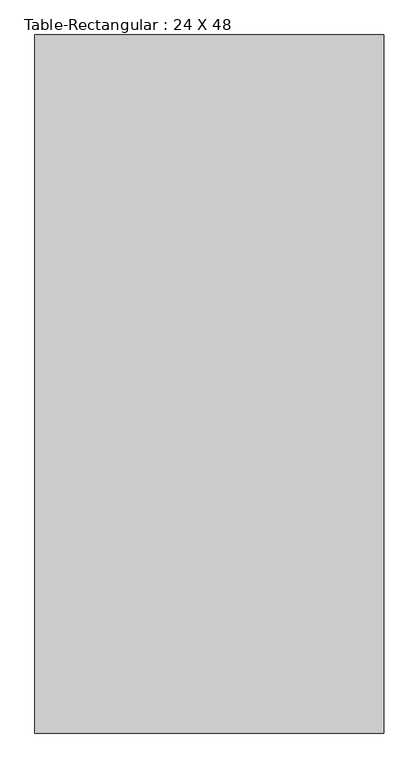
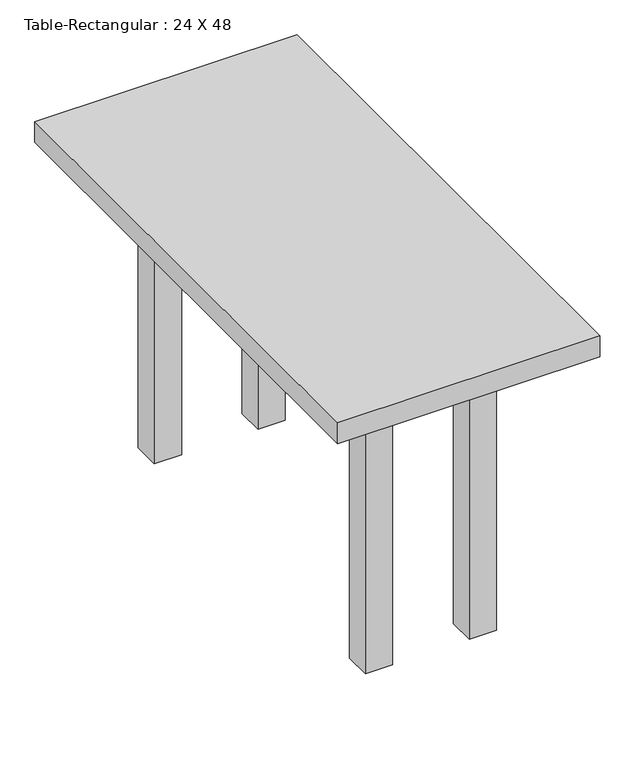
"""IFC4 building model written with IfcOpenShell, lengths in millimetres: furniture geometry, Table-Rectangular : 24 X 48."""

from ifc_helpers import new_model, si_unit, frame, origin, origin_with_axes, place, context, project, spatial, polyline, outline, extrude, source, transform, mapped, element, save


def table_rectangular_24_x_48_75328544(model_context):
    return source(origin(), model_context, "Body", "SweptSolid", [
        extrude(outline(polyline([(88.9, 419.1), (88.9, 393.7), (-88.9, 393.7), (-88.9, 419.1), (88.9, 419.1)])), frame((0.0, 0.0, 609.6), z_axis=(0.0, 0.0, 1.0), x_axis=(1.0, 0.0, 0.0)), (0.0, 0.0, 1.0), 101.6),
        extrude(outline(polyline([(88.9, -419.1), (-88.9, -419.1), (-88.9, -393.7), (88.9, -393.7), (88.9, -419.1)])), frame((0.0, 0.0, 609.6), z_axis=(0.0, 0.0, 1.0), x_axis=(1.0, 0.0, 0.0)), (0.0, 0.0, 1.0), 101.6),
        extrude(outline(polyline([(-101.6, -393.7), (-127.0, -393.7), (-127.0, 393.7), (-101.6, 393.7), (-101.6, -393.7)])), frame((0.0, 0.0, 609.6), z_axis=(0.0, 0.0, 1.0), x_axis=(1.0, 0.0, 0.0)), (0.0, 0.0, 1.0), 101.6),
        extrude(outline(polyline([(101.6, -393.7), (101.6, 393.7), (127.0, 393.7), (127.0, -393.7), (101.6, -393.7)])), frame((0.0, 0.0, 609.6), z_axis=(0.0, 0.0, 1.0), x_axis=(1.0, 0.0, 0.0)), (0.0, 0.0, 1.0), 101.6),
        extrude(outline(polyline([(304.8, 609.6), (304.8, -609.6), (-304.8, -609.6), (-304.8, 609.6), (304.8, 609.6)])), frame((0.0, 0.0, 711.2), z_axis=(0.0, 0.0, 1.0), x_axis=(1.0, 0.0, 0.0)), (0.0, 0.0, 1.0), 50.8),
        extrude(outline(polyline([(-88.9, 457.2), (-88.9, 393.7), (-152.4, 393.7), (-152.4, 457.2), (-88.9, 457.2)])), origin_with_axes(), (0.0, 0.0, 1.0), 711.2),
        extrude(outline(polyline([(88.9, 457.2), (152.4, 457.2), (152.4, 393.7), (88.9, 393.7), (88.9, 457.2)])), origin_with_axes(), (0.0, 0.0, 1.0), 711.2),
        extrude(outline(polyline([(-88.9, -457.2), (-152.4, -457.2), (-152.4, -393.7), (-88.9, -393.7), (-88.9, -457.2)])), origin_with_axes(), (0.0, 0.0, 1.0), 711.2),
        extrude(outline(polyline([(88.9, -457.2), (88.9, -393.7), (152.4, -393.7), (152.4, -457.2), (88.9, -457.2)])), origin_with_axes(), (0.0, 0.0, 1.0), 711.2),
    ])


if __name__ == "__main__":
    model = new_model("IFC4")
    model_context = context("Model", 3, world=origin())
    ifc_project = project(units=[si_unit("LENGTHUNIT", "METRE", prefix="MILLI")], contexts=[model_context])
    site = spatial("IfcSite", under=ifc_project)
    building = spatial("IfcBuilding", under=site)
    placement = place(None, origin())
    table_rectangular_24_x_48_shape = table_rectangular_24_x_48_75328544(model_context)
    element("IfcFurniture", 1, ObjectType="Table-Rectangular : 24 X 48", at=placement, inside=building, context=model_context, shape_type="MappedRepresentation", body=[
        mapped(table_rectangular_24_x_48_shape, transform((0.0, 0.0, 0.0), x_axis=(1.0, 0.0, 0.0), y_axis=(0.0, 1.0, 0.0), z_axis=(0.0, 0.0, 1.0))),
    ])
    save(model, "model.ifc")

# Revit data of these elements
# Type "Table-Rectangular : 24 X 48"
#   Assembly Code = "E2020200"
#   Height = 2' - 6"
#   Length = 2' - 0"
#   Width = 4' - 0"
#   Base Material = Wood - Birch
#   Top Material = Wood - Birch
#   Default Elevation = 0
# Element 1 (IfcFurniture, "Table-Rectangular : 24 X 48")
#   Materials on its faces: "Wood - Birch"
# Materials
#   "Wood - Birch": class "Unassigned", colour RGB 224 178 126, transparency 0
